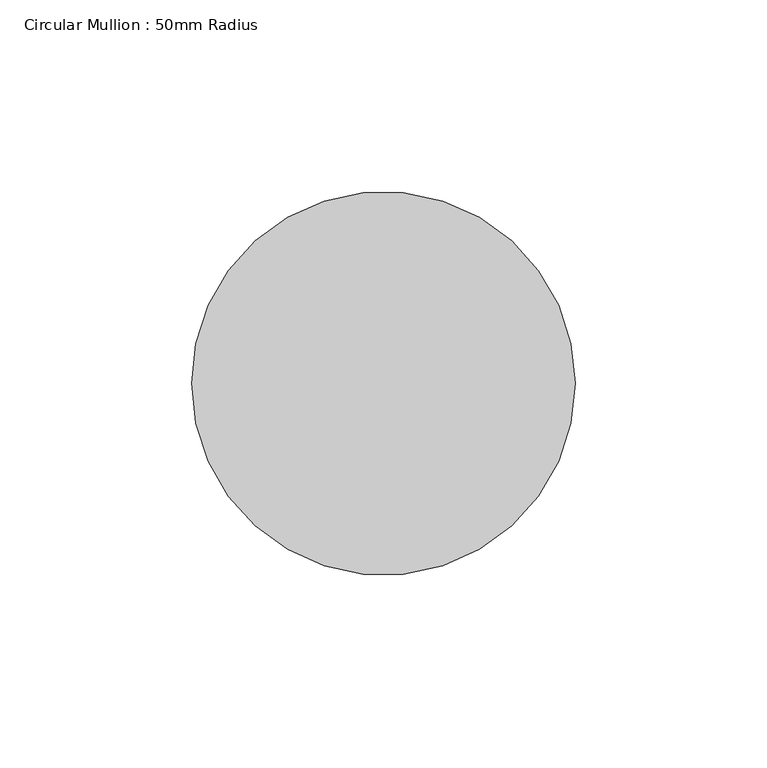
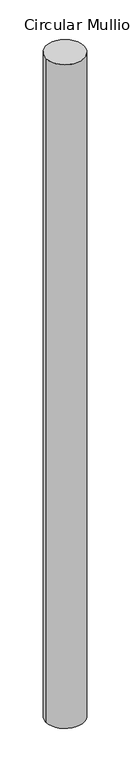
"""IFC4 building model written with IfcOpenShell, lengths in millimetres: member geometry, Circular Mullion : 50mm Radius."""

from ifc_helpers import new_model, si_unit, point, frame, origin, origin_2d, place, context, project, spatial, circle_curve, trimmed, segment, composite_curve, outline, extrude, source, transform, mapped, element, save


def circular_mullion_50mm_radius_ac85629b(model_context):
    return source(origin(), model_context, "Body", "SweptSolid", [
        extrude(outline(composite_curve([segment(trimmed(circle_curve(origin_2d(), 50.0), [point((50.0, 0.0))], [point((-50.0, 0.0))], False, "CARTESIAN"), True, "CONTINUOUS"), segment(trimmed(circle_curve(origin_2d(), 50.0), [point((-50.0, 0.0))], [point((50.0, 0.0))], False, "CARTESIAN"), True, "CONTINUOUS")], self_intersect=False)), frame((0.0, 0.0, -1843.0957728), z_axis=(0.0, 0.0, 1.0), x_axis=(1.0, 0.0, 0.0)), (0.0, 0.0, 1.0), 1843.0957728),
    ])


if __name__ == "__main__":
    model = new_model("IFC4")
    model_context = context("Model", 3, world=origin())
    ifc_project = project(units=[si_unit("LENGTHUNIT", "METRE", prefix="MILLI")], contexts=[model_context])
    site = spatial("IfcSite", under=ifc_project)
    building = spatial("IfcBuilding", under=site)
    placement = place(None, origin())
    circular_mullion_50mm_radius_shape = circular_mullion_50mm_radius_ac85629b(model_context)
    element("IfcMember", 1, ObjectType="Circular Mullion : 50mm Radius", at=placement, inside=building, context=model_context, shape_type="MappedRepresentation", body=[
        mapped(circular_mullion_50mm_radius_shape, transform((0.0, 0.0, 0.0), x_axis=(1.0, 0.0, 0.0), y_axis=(0.0, 1.0, 0.0), z_axis=(0.0, 0.0, 1.0))),
    ])
    save(model, "model.ifc")

# Revit data of these elements
# Type "Circular Mullion : 50mm Radius"
#   built-in parameter 1007350 = 0.164042 (stored number, unit not read)
# Element 1 (IfcMember, "Circular Mullion : 50mm Radius")
#   Materials on its faces: "Aluminium"
# Materials
#   "Aluminium": class "Metal", colour RGB 247 247 247, transparency 0, Description = "Aluminium 6061", Cost = 0
